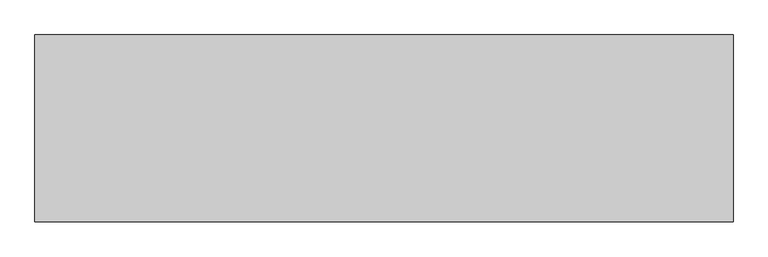
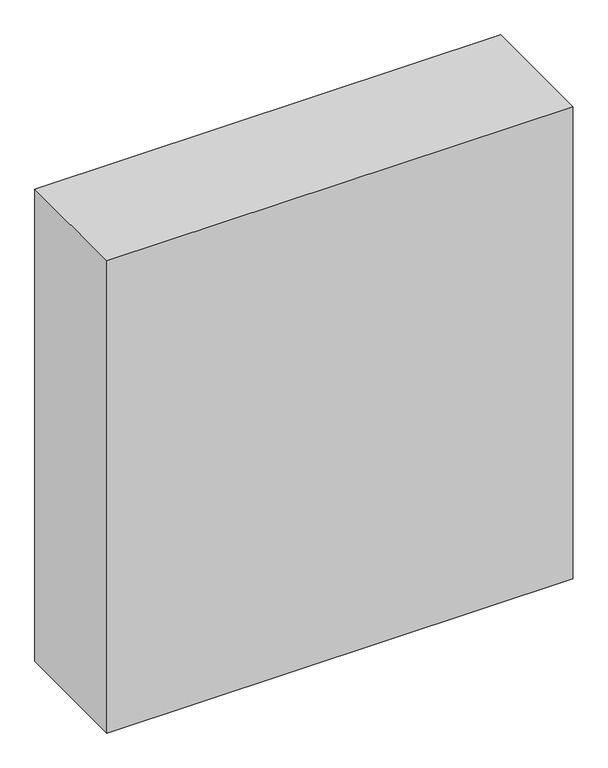
"""IFC4 building model written with IfcOpenShell, lengths in millimetres: proxy geometry, Space Planning Box_hec : Space Planning Box_hec."""

from ifc_helpers import new_model, si_unit, origin, origin_with_axes, place, context, project, spatial, polyline, outline, extrude, source, transform, mapped, element, save


def generic_models_85897e09(model_context):
    return source(origin(), model_context, "Body", "SweptSolid", [
        extrude(outline(polyline([(2800.0, 750.0), (2800.0, -750.0), (-2800.0, -750.0), (-2800.0, 750.0), (2800.0, 750.0)])), origin_with_axes(), (0.0, 0.0, 1.0), 6000.0),
    ])


if __name__ == "__main__":
    model = new_model("IFC4")
    model_context = context("Model", 3, world=origin())
    ifc_project = project(units=[si_unit("LENGTHUNIT", "METRE", prefix="MILLI")], contexts=[model_context])
    site = spatial("IfcSite", under=ifc_project)
    building = spatial("IfcBuilding", under=site)
    placement = place(None, origin())
    generic_models_shape = generic_models_85897e09(model_context)
    element("IfcBuildingElementProxy", 1, Name="Space Planning Box_hec : Space Planning Box_hec", ObjectType="Space Planning Box_hec : Space Planning Box_hec", at=placement, inside=building, context=model_context, shape_type="MappedRepresentation", body=[
        mapped(generic_models_shape, transform((0.0, 0.0, 0.0), x_axis=(1.0, 0.0, 0.0), y_axis=(0.0, 1.0, 0.0), z_axis=(0.0, 0.0, 1.0))),
    ])
    save(model, "model.ifc")

# Revit data of these elements
# Type "Space Planning Box_hec : Space Planning Box_hec"
#   Type Comments = "..."
#   Room Name [instance default] = "?"
#   Interior Finish [instance default] = ""
#   Exterior Finish [instance default] = ""
#   Department [instance default] = ""
#   Assembly Code = "..."
#   Width [instance default] = 1524 mm
#   Program Area [instance default] = 0 m²
#   Length [instance default] = 1524 mm
#   Height [instance default] = 1524 mm
#   Area [instance default] = 2.32258 m²
#   Fill Color [instance default] = Cyan
#   Default Elevation = 0
# Element 1 (IfcBuildingElementProxy, "Space Planning Box_hec : Space Planning Box_hec")
#   Room Name = "Shower Room (M)"
#   Interior Finish = "IF5"
#   Exterior Finish = "EF1"
#   Department = "AR"
#   Width = 5600 mm
#   Program Area = 31.5 m²
#   Length = 1500 mm
#   Height = 6000 mm
#   Area = 8.4 m²
#   Fill Color = Lavender
#   Materials on its faces: "Lavender"
# Materials
#   "Cyan": class "Generic", colour RGB 0 255 255, transparency 0.2, Cost = 0
#   "Lavender": class "Generic", colour RGB 186 85 211, transparency 0.2, Cost = 0
